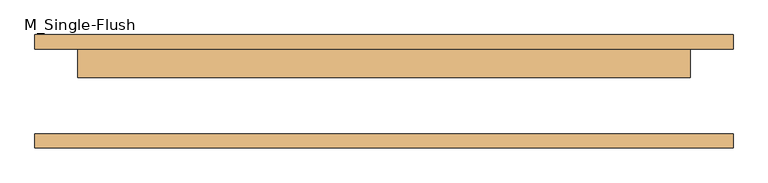
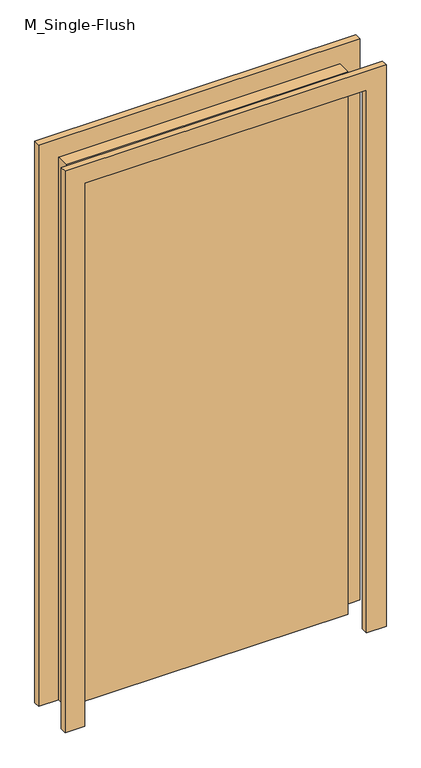
"""IFC4 building model written with IfcOpenShell, lengths in millimetres: door geometry, M_Single-Flush : Dış Kapı 1000x 2200 mm."""

from ifc_helpers import new_model, si_unit, frame, origin, origin_with_axes, place, context, project, spatial, polyline, outline, extrude, source, transform, mapped, element, save


def m_single_flush_2d738a61(model_context):
    return source(origin(), model_context, "Body", "SweptSolid", [
        extrude(outline(polyline([(2276.0, -616.0), (0.0, -616.0), (0.0, -540.0), (2200.0, -540.0), (2200.0, 540.0), (0.0, 540.0), (0.0, 616.0), (2276.0, 616.0), (2276.0, -616.0)])), frame((0.0, 75.0, 0.0), z_axis=(0.0, 1.0, 0.0), x_axis=(0.0, 0.0, 1.0)), (0.0, 0.0, 1.0), 25.0),
        extrude(outline(polyline([(2276.0, 616.0), (2276.0, -616.0), (0.0, -616.0), (0.0, -540.0), (2200.0, -540.0), (2200.0, 540.0), (0.0, 540.0), (0.0, 616.0), (2276.0, 616.0)])), frame((0.0, -100.0, 0.0), z_axis=(0.0, 1.0, 0.0), x_axis=(0.0, 0.0, 1.0)), (0.0, 0.0, 1.0), 25.0),
        extrude(outline(polyline([(540.0, 24.0), (-540.0, 24.0), (-540.0, 75.0), (540.0, 75.0), (540.0, 24.0)])), origin_with_axes(), (0.0, 0.0, 1.0), 2200.0),
    ])


if __name__ == "__main__":
    model = new_model("IFC4")
    model_context = context("Model", 3, world=origin())
    ifc_project = project(units=[si_unit("LENGTHUNIT", "METRE", prefix="MILLI")], contexts=[model_context])
    site = spatial("IfcSite", under=ifc_project)
    building = spatial("IfcBuilding", under=site)
    placement = place(None, origin())
    m_single_flush_shape = m_single_flush_2d738a61(model_context)
    element("IfcDoor", 1, ObjectType="M_Single-Flush : Dış Kapı 1000x 2200 mm", at=placement, inside=building, context=model_context, shape_type="MappedRepresentation", body=[
        mapped(m_single_flush_shape, transform((0.0, 0.0, 0.0), x_axis=(1.0, 0.0, 0.0), y_axis=(0.0, 1.0, 0.0), z_axis=(0.0, 0.0, 1.0))),
    ])
    save(model, "model.ifc")

# Revit data of these elements
# Type "M_Single-Flush : Dış Kapı 1000x 2200 mm"
#   Type Mark = "23"
#   Construction Type Id = "MDOOR"
#   Analytic Construction = "Metal"
#   Thickness = 5.1 cm
#   Thermal Resistance (R) = 0.270117 (m²·K)/W
#   Heat Transfer Coefficient (U) = 3.7021 W/(m²·K)
#   Height = 220 cm
#   Trim Projection Ext = 2.5 cm
#   Trim Projection Int = 2.5 cm
#   Trim Width = 7.6 cm
#   Width = 108 cm
#   Define Thermal Properties by = 1
#   Door Material = Door - Panel
#   Frame Material = Door - Frame
#   Visual Light Transmittance = 0
#   Solar Heat Gain Coefficient = 0
#   Function = (empty or 0)
#   Wall Closure = (empty or 0)
# Element 1 (IfcDoor, "M_Single-Flush : Dış Kapı 1000x 2200 mm")
#   Materials on its faces: "Door - Frame", "Door - Panel"
# Materials
#   "Door - Panel": class "Wood", colour RGB 210 159 95, transparency 0, Cost = 0
#   "Door - Frame": class "Miscellaneous", colour RGB 118 70 51, transparency 0, Cost = 0
